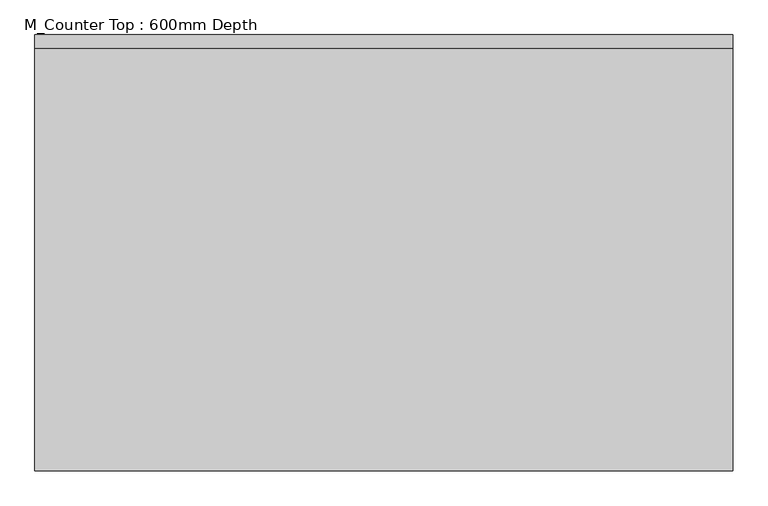
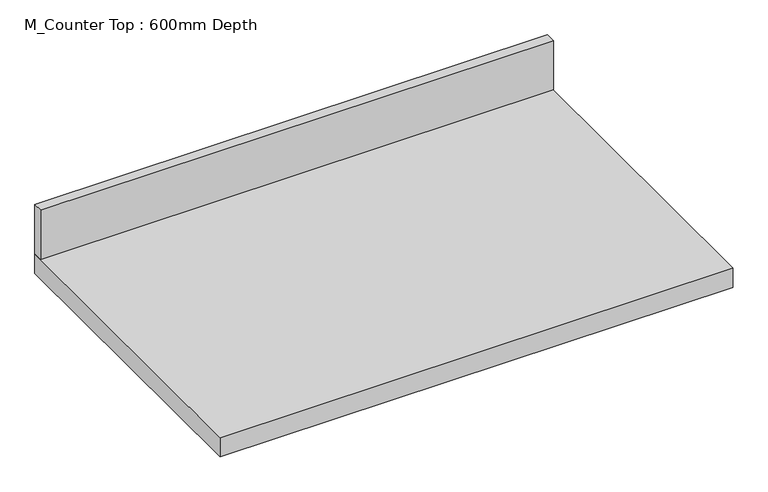
"""IFC4 building model written with IfcOpenShell, lengths in millimetres: furniture geometry, M_Counter Top : 600mm Depth."""

import ifcopenshell
import ifcopenshell.guid

model = None  # the IFC model being written
_history = None  # IfcOwnerHistory: only IFC2X3 demands one
_inside = {}  # id of a spatial element -> (the spatial element, [elements in it])
_under = {}  # id of a project, library or spatial element -> (it, [spatial elements below it])
_declared = {}  # id of a project -> (the project, [libraries it declares])
_typed = {}  # id of a type object -> (the type object, [elements of that type])
_made_of = {}  # id of a material, layer set ... -> (it, [elements and type objects made of it])


def new_model(schema):
    """Start an empty IFC model of exactly this schema.

    Asked for "IFC4X3", IfcOpenShell would pick the latest addendum, in which some entities
    have other attributes; the version numbers below select the first issue.
    IFC2X3 requires an IfcOwnerHistory on every rooted entity: one is made here for all.
    """
    global model, _history
    if schema == "IFC4X3":
        model = ifcopenshell.file(schema_version=(4, 3, 0, 0))
    else:
        model = ifcopenshell.file(schema=schema)
    _inside.clear()
    _under.clear()
    _declared.clear()
    _typed.clear()
    _made_of.clear()
    _history = None
    if model.schema == "IFC2X3":
        org = make("IfcOrganization", Name="unknown")
        user = make(
            "IfcPersonAndOrganization",
            ThePerson=make("IfcPerson", FamilyName="unknown"),
            TheOrganization=org,
        )
        app = make(
            "IfcApplication",
            ApplicationDeveloper=org,
            Version="unknown",
            ApplicationFullName="unknown",
            ApplicationIdentifier="unknown",
        )
        _history = make(
            "IfcOwnerHistory",
            OwningUser=user,
            OwningApplication=app,
            ChangeAction="ADDED",
            CreationDate=0,
        )
    return model


def make(cls, **values):
    """One entity of the class cls with the attributes given. An attribute that is None is left unset."""
    return model.create_entity(
        cls, **{name: value for name, value in values.items() if value is not None}
    )


def rooted(cls, **values):
    """An entity with a GlobalId (a new one), such as an element, a storey or a relation."""
    return make(cls, GlobalId=ifcopenshell.guid.new(), OwnerHistory=_history, **values)


def si_unit(unit_type, name, prefix=None):
    """IfcSIUnit, for example si_unit("LENGTHUNIT", "METRE", prefix="MILLI")."""
    return make("IfcSIUnit", UnitType=unit_type, Prefix=prefix, Name=name)


def assignment(units):
    """IfcUnitAssignment: the units of a project."""
    return None if units is None else make("IfcUnitAssignment", Units=units)


def point(xyz):
    """IfcCartesianPoint."""
    return None if xyz is None else make("IfcCartesianPoint", Coordinates=xyz)


def direction(xyz):
    """IfcDirection."""
    return None if xyz is None else make("IfcDirection", DirectionRatios=xyz)


def frame(location, z_axis=None, x_axis=None):
    """IfcAxis2Placement3D, a coordinate frame: its origin and axes. An axis left out is left unset."""
    return make(
        "IfcAxis2Placement3D",
        Location=point(location),
        Axis=direction(z_axis),
        RefDirection=direction(x_axis),
    )


def origin():
    """The frame at (0, 0, 0) with its axes left unset."""
    return frame((0.0, 0.0, 0.0))


def place(relative_to, where):
    """IfcLocalPlacement: puts the frame where relative to a parent placement (None: the world)."""
    return make(
        "IfcLocalPlacement", PlacementRelTo=relative_to, RelativePlacement=where
    )


def context(
    kind, dimensions, precision=None, world=None, true_north=None, identifier=None
):
    """IfcGeometricRepresentationContext, for example the 3D "Model" context."""
    return make(
        "IfcGeometricRepresentationContext",
        ContextIdentifier=identifier,
        ContextType=kind,
        CoordinateSpaceDimension=dimensions,
        Precision=precision,
        WorldCoordinateSystem=world,
        TrueNorth=true_north,
    )


def project(units=None, contexts=None):
    """IfcProject with its units and contexts."""
    return rooted(
        "IfcProject",
        Name="project",
        RepresentationContexts=contexts,
        UnitsInContext=assignment(units),
    )


def spatial(cls, under=None, at=None, **own):
    """A site, building, storey or space (cls), placed at a placement, below another one or the project."""
    s = rooted(cls, ObjectPlacement=at, **own)
    if under is not None:
        _under.setdefault(under.id(), (under, []))[1].append(s)
    return s


def polyline(points):
    """IfcPolyline through the points."""
    return make("IfcPolyline", Points=[point(p) for p in points])


def outline(outer, holes=None, kind="AREA"):
    """IfcArbitraryClosedProfileDef: a profile drawn as a closed curve; with holes, ...WithVoids."""
    if holes is None:
        return make("IfcArbitraryClosedProfileDef", ProfileType=kind, OuterCurve=outer)
    return make(
        "IfcArbitraryProfileDefWithVoids",
        ProfileType=kind,
        OuterCurve=outer,
        InnerCurves=holes,
    )


def extrude(swept, where, along, depth):
    """IfcExtrudedAreaSolid: the profile swept, set in the frame where, extruded along a direction by depth."""
    return make(
        "IfcExtrudedAreaSolid",
        SweptArea=swept,
        Position=where,
        ExtrudedDirection=direction(along),
        Depth=depth,
    )


def shape(context_of_items, identifier, shape_type, items):
    """IfcShapeRepresentation: the items that make up one representation, for example the "Body"."""
    return make(
        "IfcShapeRepresentation",
        ContextOfItems=context_of_items,
        RepresentationIdentifier=identifier,
        RepresentationType=shape_type,
        Items=items,
    )


def source(mapping_origin, context_of_items, identifier, shape_type, items):
    """IfcRepresentationMap: a shape defined once, which mapped items show again and again."""
    return make(
        "IfcRepresentationMap",
        MappingOrigin=mapping_origin,
        MappedRepresentation=shape(context_of_items, identifier, shape_type, items),
    )


def transform(
    local_origin,
    x_axis=None,
    y_axis=None,
    z_axis=None,
    scale=None,
    scale2=None,
    scale3=None,
    uniform=True,
):
    """IfcCartesianTransformationOperator3D, or its non-uniform kind. x_axis, y_axis, z_axis: its Axis1, 2, 3."""
    if uniform:
        return make(
            "IfcCartesianTransformationOperator3D",
            Axis1=direction(x_axis),
            Axis2=direction(y_axis),
            LocalOrigin=point(local_origin),
            Scale=scale,
            Axis3=direction(z_axis),
        )
    return make(
        "IfcCartesianTransformationOperator3DnonUniform",
        Axis1=direction(x_axis),
        Axis2=direction(y_axis),
        LocalOrigin=point(local_origin),
        Scale=scale,
        Axis3=direction(z_axis),
        Scale2=scale2,
        Scale3=scale3,
    )


def mapped(mapping_source, mapping_target):
    """IfcMappedItem: shows the shape of a source again, moved by a transform."""
    return make(
        "IfcMappedItem", MappingSource=mapping_source, MappingTarget=mapping_target
    )


def made_of(thing, what):
    """Note that an element or type object is made of a material, layer set ...; save() writes the relation."""
    if what is not None:
        _made_of.setdefault(what.id(), (what, []))[1].append(thing)
    return thing


def element(
    cls,
    number,
    at=None,
    inside=None,
    cuts=None,
    type_object=None,
    material=None,
    context=None,
    identifier="Body",
    shape_type=None,
    held_by="IfcProductDefinitionShape",
    body=None,
    shapes=None,
    **own,
):
    """One element of the class cls, such as IfcWall. Its Tag is "e" and its number.

    at: its placement. inside: the storey or other place that contains it. cuts: it is an
    opening in that element (IfcRelVoidsElement). A single representation is given by context,
    identifier, shape_type and body (its items); several are given by shapes. held_by: the class
    of the entity that holds the representations. save() writes the other relations.
    """
    e = rooted(cls, Tag="e%d" % number, ObjectPlacement=at, **own)
    if body is not None:
        shapes = [shape(context, identifier, shape_type, body)]
    if shapes is not None:
        e.Representation = make(held_by, Representations=shapes)
    if inside is not None:
        _inside.setdefault(inside.id(), (inside, []))[1].append(e)
    if cuts is not None:
        rooted(
            "IfcRelVoidsElement", RelatingBuildingElement=cuts, RelatedOpeningElement=e
        )
    if type_object is not None:
        _typed.setdefault(type_object.id(), (type_object, []))[1].append(e)
    return made_of(e, material)


def aggregate(whole, parts):
    """IfcRelAggregates: a whole, such as a stair, and the parts it consists of."""
    return rooted("IfcRelAggregates", RelatingObject=whole, RelatedObjects=parts)


def save(model, path):
    """Write the relations noted so far, then the file.

    IfcRelAggregates (storeys below a building ...), IfcRelContainedInSpatialStructure (elements
    in a storey), IfcRelDefinesByType, IfcRelAssociatesMaterial and IfcRelDeclares: one each for
    every whole, place, type object, material and project.
    """
    for whole, parts in _under.values():
        aggregate(whole, parts)
    for where, things in _inside.values():
        rooted(
            "IfcRelContainedInSpatialStructure",
            RelatedElements=things,
            RelatingStructure=where,
        )
    for kind, things in _typed.values():
        rooted("IfcRelDefinesByType", RelatedObjects=things, RelatingType=kind)
    for what, things in _made_of.values():
        rooted("IfcRelAssociatesMaterial", RelatedObjects=things, RelatingMaterial=what)
    for by, libraries in _declared.values():
        rooted("IfcRelDeclares", RelatingContext=by, RelatedDefinitions=libraries)
    model.write(path)


def m_counter_top_600mm_depth_0fb62e5d(model_context):
    return source(origin(), model_context, "Body", "SweptSolid", [
        extrude(outline(polyline([(-1200.4622951, 0.0), (-200.4622951, 0.0), (-200.4622951, -19.05), (-1200.4622951, -19.05), (-1200.4622951, 0.0)])), frame((0.0, 0.0, 900.0), z_axis=(0.0, 0.0, 1.0), x_axis=(1.0, 0.0, 0.0)), (0.0, 0.0, 1.0), 101.6),
        extrude(outline(polyline([(-200.4622951, 0.0), (-200.4622951, -625.0), (-1200.4622951, -625.0), (-1200.4622951, 0.0), (-200.4622951, 0.0)])), frame((0.0, 0.0, 860.0), z_axis=(0.0, 0.0, 1.0), x_axis=(1.0, 0.0, 0.0)), (0.0, 0.0, 1.0), 40.0),
    ])


if __name__ == "__main__":
    model = new_model("IFC4")
    model_context = context("Model", 3, world=origin())
    ifc_project = project(units=[si_unit("LENGTHUNIT", "METRE", prefix="MILLI")], contexts=[model_context])
    site = spatial("IfcSite", under=ifc_project)
    building = spatial("IfcBuilding", under=site)
    placement = place(None, origin())
    m_counter_top_600mm_depth_shape = m_counter_top_600mm_depth_0fb62e5d(model_context)
    element("IfcFurniture", 1, ObjectType="M_Counter Top : 600mm Depth", at=placement, inside=building, context=model_context, shape_type="MappedRepresentation", body=[
        mapped(m_counter_top_600mm_depth_shape, transform((0.0, 0.0, 0.0), x_axis=(1.0, 0.0, 0.0), y_axis=(0.0, 1.0, 0.0), z_axis=(0.0, 0.0, 1.0))),
    ])
    save(model, "model.ifc")

# Revit data of these elements
# Type "M_Counter Top : 600mm Depth"
#   AccessibilityPerformance = "AccessibilityPerformance"
#   CodePerformance = "CodePerformance"
#   Area = "Area"
#   Color = "Color"
#   Constituents = "Constituents"
#   Features = "Features"
#   Finish = "Finish"
#   Grade = "Grade"
#   Material = "Material"
#   ModelReference = "ModelReference"
#   NominalHeight = "NominalHeight"
#   NominalLength = "NominalLength"
#   NominalWidth = "NominalWidth"
#   ProductionYear = "ProductionYear"
#   Reference = "Reference"
#   Shape = "Shape"
#   Size = "Size"
#   SustainabilityPerformance = "SustainabilityPerformance"
#   WarrantyDescription = "WarrantyDescription"
#   WarrantyDurationLabor = "WarrantyDurationLabor"
#   WarrantyDurationParts = "WarrantyDurationParts"
#   WarrantyGuarantorLabor = "WarrantyGuarantorLabor"
#   WarrantyGuarantorParts = "WarrantyGuarantorParts"
#   ExpectedLife = "ExpectedLife"
#   ReplacementCost = "ReplacementCost"
#   AssetAccountingType = "FIXED"
#   ModelLabel = "ModelLabel"
#   Manufacturer = "Manufacturer"
#   Finish = "Finish"
#   Construction Type = "Construction Type"
#   Counter Thickness = 0.040 m
#   Depth = 0.625 m
#   Height = 0.900 m
#   Length [instance default] = 2.500 m
#   Backsplash Visibility [instance default] = yes
#   Counter Top Material = none
#   Assembly Code = ""
# Element 1 (IfcFurniture, "M_Counter Top : 600mm Depth")
#   Length = 1.000 m
#   Materials on its faces: "Counter Top"
# Materials
#   "Counter Top": class "Wood", colour RGB 226 177 128, transparency 0
